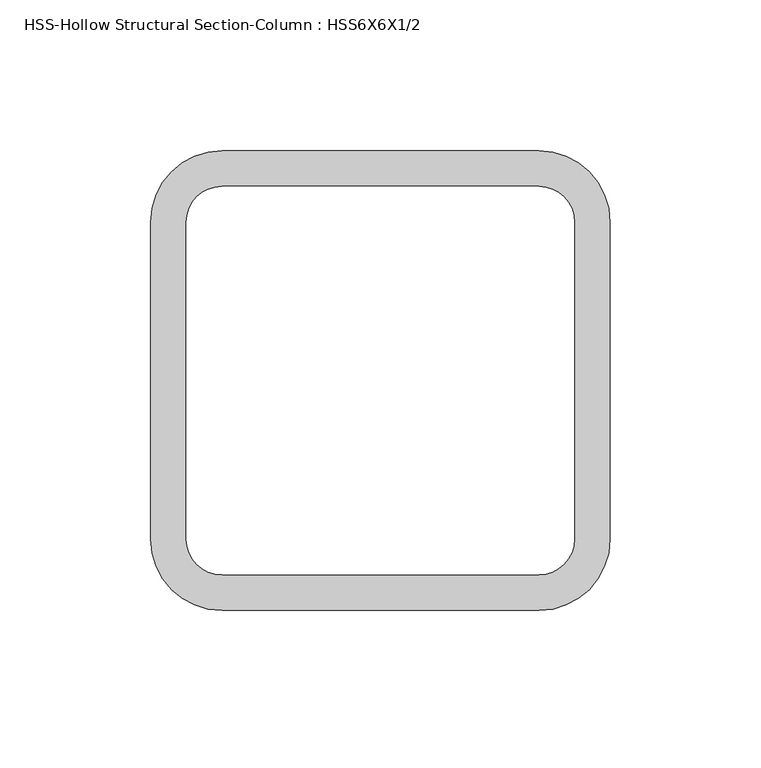
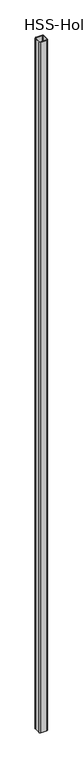
"""IFC4 building model written with IfcOpenShell, lengths in millimetres: column geometry, HSS-Hollow Structural Section-Column : HSS6X6X1/2."""

from ifc_helpers import new_model, si_unit, point, frame, frame_2d, origin, place, context, project, spatial, polyline, circle_curve, trimmed, segment, composite_curve, outline, extrude, source, transform, mapped, element, save


def hss_hollow_structural_section_column_hss6x6x1_2_8becbb64(model_context):
    return source(origin(), model_context, "Body", "SweptSolid", [
        extrude(outline(composite_curve([segment(trimmed(circle_curve(frame_2d((52.578, 52.578)), 23.622), [point((52.578, 76.2))], [point((76.2, 52.578))], False, "CARTESIAN"), True, "CONTINUOUS"), segment(polyline([(76.2, 52.578), (76.2, -52.578)]), True, "CONTINUOUS"), segment(trimmed(circle_curve(frame_2d((52.578, -52.578)), 23.622), [point((76.2, -52.578))], [point((52.578, -76.2))], False, "CARTESIAN"), True, "CONTINUOUS"), segment(polyline([(52.578, -76.2), (-52.578, -76.2)]), True, "CONTINUOUS"), segment(trimmed(circle_curve(frame_2d((-52.578, -52.578)), 23.622), [point((-52.578, -76.2))], [point((-76.2, -52.578))], False, "CARTESIAN"), True, "CONTINUOUS"), segment(polyline([(-76.2, -52.578), (-76.2, 52.578)]), True, "CONTINUOUS"), segment(trimmed(circle_curve(frame_2d((-52.578, 52.578)), 23.622), [point((-76.2, 52.578))], [point((-52.578, 76.2))], False, "CARTESIAN"), True, "CONTINUOUS"), segment(polyline([(-52.578, 76.2), (52.578, 76.2)]), True, "CONTINUOUS")], self_intersect=False), holes=[composite_curve([segment(polyline([(52.578, 64.389), (-52.578, 64.389)]), True, "CONTINUOUS"), segment(trimmed(circle_curve(frame_2d((-52.578, 52.578)), 11.811), [point((-52.578, 64.389))], [point((-64.389, 52.578))], True, "CARTESIAN"), True, "CONTINUOUS"), segment(polyline([(-64.389, 52.578), (-64.389, -52.578)]), True, "CONTINUOUS"), segment(trimmed(circle_curve(frame_2d((-52.578, -52.578)), 11.811), [point((-64.389, -52.578))], [point((-52.578, -64.389))], True, "CARTESIAN"), True, "CONTINUOUS"), segment(polyline([(-52.578, -64.389), (52.578, -64.389)]), True, "CONTINUOUS"), segment(trimmed(circle_curve(frame_2d((52.578, -52.578)), 11.811), [point((52.578, -64.389))], [point((64.389, -52.578))], True, "CARTESIAN"), True, "CONTINUOUS"), segment(polyline([(64.389, -52.578), (64.389, 52.578)]), True, "CONTINUOUS"), segment(trimmed(circle_curve(frame_2d((52.578, 52.578)), 11.811), [point((64.389, 52.578))], [point((52.578, 64.389))], True, "CARTESIAN"), True, "CONTINUOUS")], self_intersect=False)]), frame((0.0, 0.0, -609.6), z_axis=(0.0, 0.0, 1.0), x_axis=(1.0, 0.0, 0.0)), (0.0, 0.0, 1.0), 12954.0),
    ])


if __name__ == "__main__":
    model = new_model("IFC4")
    model_context = context("Model", 3, world=origin())
    ifc_project = project(units=[si_unit("LENGTHUNIT", "METRE", prefix="MILLI")], contexts=[model_context])
    site = spatial("IfcSite", under=ifc_project)
    building = spatial("IfcBuilding", under=site)
    placement = place(None, origin())
    hss_hollow_structural_section_column_hss6x6x1_2_shape = hss_hollow_structural_section_column_hss6x6x1_2_8becbb64(model_context)
    element("IfcColumn", 1, ObjectType="HSS-Hollow Structural Section-Column : HSS6X6X1/2", at=placement, inside=building, context=model_context, shape_type="MappedRepresentation", body=[
        mapped(hss_hollow_structural_section_column_hss6x6x1_2_shape, transform((0.0, 0.0, 0.0), x_axis=(1.0, 0.0, 0.0), y_axis=(0.0, 1.0, 0.0), z_axis=(0.0, 0.0, 1.0))),
    ])
    save(model, "model.ifc")

# Revit data of these elements
# Type "HSS-Hollow Structural Section-Column : HSS6X6X1/2"
#   Assembly Code = "B10"
#   Shape = "Square"
#   W = 35.1
#   Ht = 0' - 6"
#   b = 0' - 6"
#   kr = 0' - 0.93"
#   t = 0' - 0.465"
#   A = 0.0676389 SF
#   Structural Material [instance default] = Steel ASTM A500, Grade B, Rectangular and Square
# Element 1 (IfcColumn, "HSS-Hollow Structural Section-Column : HSS6X6X1/2")
#   Materials on its faces: "Steel ASTM A500, Grade B, Rectangular and Square"
# Materials
#   "Steel ASTM A500, Grade B, Rectangular and Square": class "Metal", colour RGB 199 199 199, transparency 0, Description = "Carbon steel", Cost = 0
